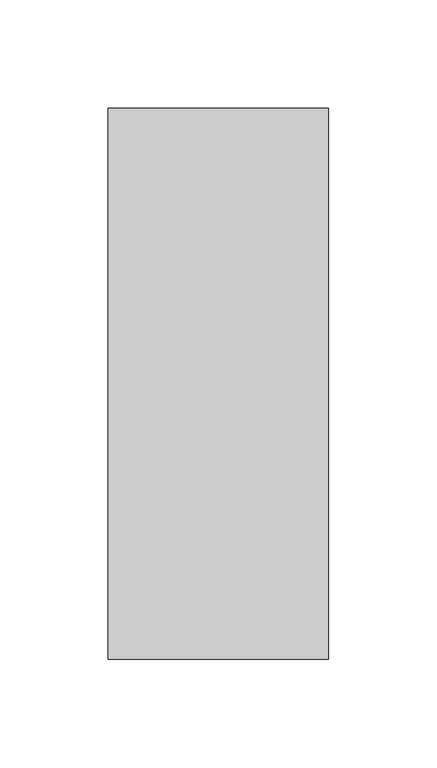
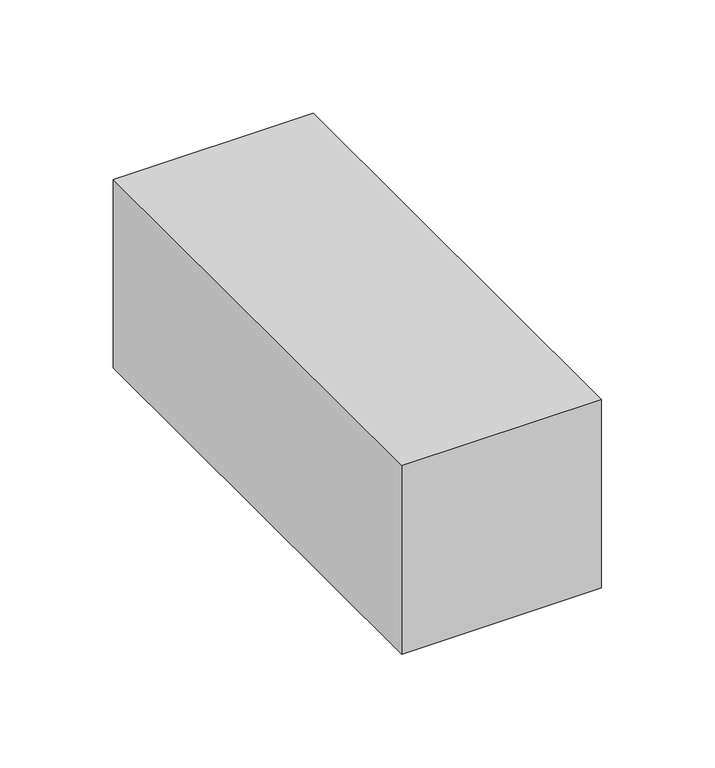
"""IFC4 building model written with IfcOpenShell, lengths in millimetres: proxy geometry, M0750 - Flowmeter, Air, Connect W50 PSI Supply : M0750 - Flowmeter, Air, Connect W50 PSI Supply."""

import ifcopenshell
import ifcopenshell.guid

model = None  # the IFC model being written
_history = None  # IfcOwnerHistory: only IFC2X3 demands one
_inside = {}  # id of a spatial element -> (the spatial element, [elements in it])
_under = {}  # id of a project, library or spatial element -> (it, [spatial elements below it])
_declared = {}  # id of a project -> (the project, [libraries it declares])
_typed = {}  # id of a type object -> (the type object, [elements of that type])
_made_of = {}  # id of a material, layer set ... -> (it, [elements and type objects made of it])


def new_model(schema):
    """Start an empty IFC model of exactly this schema.

    Asked for "IFC4X3", IfcOpenShell would pick the latest addendum, in which some entities
    have other attributes; the version numbers below select the first issue.
    IFC2X3 requires an IfcOwnerHistory on every rooted entity: one is made here for all.
    """
    global model, _history
    if schema == "IFC4X3":
        model = ifcopenshell.file(schema_version=(4, 3, 0, 0))
    else:
        model = ifcopenshell.file(schema=schema)
    _inside.clear()
    _under.clear()
    _declared.clear()
    _typed.clear()
    _made_of.clear()
    _history = None
    if model.schema == "IFC2X3":
        org = make("IfcOrganization", Name="unknown")
        user = make(
            "IfcPersonAndOrganization",
            ThePerson=make("IfcPerson", FamilyName="unknown"),
            TheOrganization=org,
        )
        app = make(
            "IfcApplication",
            ApplicationDeveloper=org,
            Version="unknown",
            ApplicationFullName="unknown",
            ApplicationIdentifier="unknown",
        )
        _history = make(
            "IfcOwnerHistory",
            OwningUser=user,
            OwningApplication=app,
            ChangeAction="ADDED",
            CreationDate=0,
        )
    return model


def make(cls, **values):
    """One entity of the class cls with the attributes given. An attribute that is None is left unset."""
    return model.create_entity(
        cls, **{name: value for name, value in values.items() if value is not None}
    )


def rooted(cls, **values):
    """An entity with a GlobalId (a new one), such as an element, a storey or a relation."""
    return make(cls, GlobalId=ifcopenshell.guid.new(), OwnerHistory=_history, **values)


def si_unit(unit_type, name, prefix=None):
    """IfcSIUnit, for example si_unit("LENGTHUNIT", "METRE", prefix="MILLI")."""
    return make("IfcSIUnit", UnitType=unit_type, Prefix=prefix, Name=name)


def assignment(units):
    """IfcUnitAssignment: the units of a project."""
    return None if units is None else make("IfcUnitAssignment", Units=units)


def point(xyz):
    """IfcCartesianPoint."""
    return None if xyz is None else make("IfcCartesianPoint", Coordinates=xyz)


def direction(xyz):
    """IfcDirection."""
    return None if xyz is None else make("IfcDirection", DirectionRatios=xyz)


def frame(location, z_axis=None, x_axis=None):
    """IfcAxis2Placement3D, a coordinate frame: its origin and axes. An axis left out is left unset."""
    return make(
        "IfcAxis2Placement3D",
        Location=point(location),
        Axis=direction(z_axis),
        RefDirection=direction(x_axis),
    )


def frame_2d(location, x_axis=None):
    """IfcAxis2Placement2D, a coordinate frame in the plane: its origin and x axis."""
    return make(
        "IfcAxis2Placement2D", Location=point(location), RefDirection=direction(x_axis)
    )


def origin():
    """The frame at (0, 0, 0) with its axes left unset."""
    return frame((0.0, 0.0, 0.0))


def origin_with_axes():
    """The frame at (0, 0, 0) with the z axis (0, 0, 1) and the x axis (1, 0, 0) written out."""
    return frame((0.0, 0.0, 0.0), z_axis=(0.0, 0.0, 1.0), x_axis=(1.0, 0.0, 0.0))


def place(relative_to, where):
    """IfcLocalPlacement: puts the frame where relative to a parent placement (None: the world)."""
    return make(
        "IfcLocalPlacement", PlacementRelTo=relative_to, RelativePlacement=where
    )


def context(
    kind, dimensions, precision=None, world=None, true_north=None, identifier=None
):
    """IfcGeometricRepresentationContext, for example the 3D "Model" context."""
    return make(
        "IfcGeometricRepresentationContext",
        ContextIdentifier=identifier,
        ContextType=kind,
        CoordinateSpaceDimension=dimensions,
        Precision=precision,
        WorldCoordinateSystem=world,
        TrueNorth=true_north,
    )


def project(units=None, contexts=None):
    """IfcProject with its units and contexts."""
    return rooted(
        "IfcProject",
        Name="project",
        RepresentationContexts=contexts,
        UnitsInContext=assignment(units),
    )


def spatial(cls, under=None, at=None, **own):
    """A site, building, storey or space (cls), placed at a placement, below another one or the project."""
    s = rooted(cls, ObjectPlacement=at, **own)
    if under is not None:
        _under.setdefault(under.id(), (under, []))[1].append(s)
    return s


def polyline(points):
    """IfcPolyline through the points."""
    return make("IfcPolyline", Points=[point(p) for p in points])


def circle_curve(where, radius):
    """IfcCircle in the frame where."""
    return make("IfcCircle", Position=where, Radius=radius)


def trimmed(basis, trim1, trim2, sense, master):
    """IfcTrimmedCurve: the piece of a basis curve between two trims."""
    return make(
        "IfcTrimmedCurve",
        BasisCurve=basis,
        Trim1=trim1,
        Trim2=trim2,
        SenseAgreement=sense,
        MasterRepresentation=master,
    )


def segment(curve, same_sense, transition):
    """IfcCompositeCurveSegment."""
    return make(
        "IfcCompositeCurveSegment",
        Transition=transition,
        SameSense=same_sense,
        ParentCurve=curve,
    )


def composite_curve(segments, self_intersect=None):
    """IfcCompositeCurve: segments joined end to end."""
    return make("IfcCompositeCurve", Segments=segments, SelfIntersect=self_intersect)


def outline(outer, holes=None, kind="AREA"):
    """IfcArbitraryClosedProfileDef: a profile drawn as a closed curve; with holes, ...WithVoids."""
    if holes is None:
        return make("IfcArbitraryClosedProfileDef", ProfileType=kind, OuterCurve=outer)
    return make(
        "IfcArbitraryProfileDefWithVoids",
        ProfileType=kind,
        OuterCurve=outer,
        InnerCurves=holes,
    )


def extrude(swept, where, along, depth):
    """IfcExtrudedAreaSolid: the profile swept, set in the frame where, extruded along a direction by depth."""
    return make(
        "IfcExtrudedAreaSolid",
        SweptArea=swept,
        Position=where,
        ExtrudedDirection=direction(along),
        Depth=depth,
    )


def shape(context_of_items, identifier, shape_type, items):
    """IfcShapeRepresentation: the items that make up one representation, for example the "Body"."""
    return make(
        "IfcShapeRepresentation",
        ContextOfItems=context_of_items,
        RepresentationIdentifier=identifier,
        RepresentationType=shape_type,
        Items=items,
    )


def source(mapping_origin, context_of_items, identifier, shape_type, items):
    """IfcRepresentationMap: a shape defined once, which mapped items show again and again."""
    return make(
        "IfcRepresentationMap",
        MappingOrigin=mapping_origin,
        MappedRepresentation=shape(context_of_items, identifier, shape_type, items),
    )


def transform(
    local_origin,
    x_axis=None,
    y_axis=None,
    z_axis=None,
    scale=None,
    scale2=None,
    scale3=None,
    uniform=True,
):
    """IfcCartesianTransformationOperator3D, or its non-uniform kind. x_axis, y_axis, z_axis: its Axis1, 2, 3."""
    if uniform:
        return make(
            "IfcCartesianTransformationOperator3D",
            Axis1=direction(x_axis),
            Axis2=direction(y_axis),
            LocalOrigin=point(local_origin),
            Scale=scale,
            Axis3=direction(z_axis),
        )
    return make(
        "IfcCartesianTransformationOperator3DnonUniform",
        Axis1=direction(x_axis),
        Axis2=direction(y_axis),
        LocalOrigin=point(local_origin),
        Scale=scale,
        Axis3=direction(z_axis),
        Scale2=scale2,
        Scale3=scale3,
    )


def mapped(mapping_source, mapping_target):
    """IfcMappedItem: shows the shape of a source again, moved by a transform."""
    return make(
        "IfcMappedItem", MappingSource=mapping_source, MappingTarget=mapping_target
    )


def made_of(thing, what):
    """Note that an element or type object is made of a material, layer set ...; save() writes the relation."""
    if what is not None:
        _made_of.setdefault(what.id(), (what, []))[1].append(thing)
    return thing


def element(
    cls,
    number,
    at=None,
    inside=None,
    cuts=None,
    type_object=None,
    material=None,
    context=None,
    identifier="Body",
    shape_type=None,
    held_by="IfcProductDefinitionShape",
    body=None,
    shapes=None,
    **own,
):
    """One element of the class cls, such as IfcWall. Its Tag is "e" and its number.

    at: its placement. inside: the storey or other place that contains it. cuts: it is an
    opening in that element (IfcRelVoidsElement). A single representation is given by context,
    identifier, shape_type and body (its items); several are given by shapes. held_by: the class
    of the entity that holds the representations. save() writes the other relations.
    """
    e = rooted(cls, Tag="e%d" % number, ObjectPlacement=at, **own)
    if body is not None:
        shapes = [shape(context, identifier, shape_type, body)]
    if shapes is not None:
        e.Representation = make(held_by, Representations=shapes)
    if inside is not None:
        _inside.setdefault(inside.id(), (inside, []))[1].append(e)
    if cuts is not None:
        rooted(
            "IfcRelVoidsElement", RelatingBuildingElement=cuts, RelatedOpeningElement=e
        )
    if type_object is not None:
        _typed.setdefault(type_object.id(), (type_object, []))[1].append(e)
    return made_of(e, material)


def aggregate(whole, parts):
    """IfcRelAggregates: a whole, such as a stair, and the parts it consists of."""
    return rooted("IfcRelAggregates", RelatingObject=whole, RelatedObjects=parts)


def save(model, path):
    """Write the relations noted so far, then the file.

    IfcRelAggregates (storeys below a building ...), IfcRelContainedInSpatialStructure (elements
    in a storey), IfcRelDefinesByType, IfcRelAssociatesMaterial and IfcRelDeclares: one each for
    every whole, place, type object, material and project.
    """
    for whole, parts in _under.values():
        aggregate(whole, parts)
    for where, things in _inside.values():
        rooted(
            "IfcRelContainedInSpatialStructure",
            RelatedElements=things,
            RelatingStructure=where,
        )
    for kind, things in _typed.values():
        rooted("IfcRelDefinesByType", RelatedObjects=things, RelatingType=kind)
    for what, things in _made_of.values():
        rooted("IfcRelAssociatesMaterial", RelatedObjects=things, RelatingMaterial=what)
    for by, libraries in _declared.values():
        rooted("IfcRelDeclares", RelatingContext=by, RelatedDefinitions=libraries)
    model.write(path)


def plane_surface(at):
    """IfcPlane: the flat surface through the origin of the frame at, square to its z axis."""
    return make("IfcPlane", Position=at)


def cylinder_surface(at, radius):
    """IfcCylindricalSurface: all points at the distance radius from the z axis of the frame at."""
    return make("IfcCylindricalSurface", Position=at, Radius=radius)


def revolved_surface(curve, axis_point, axis_direction):
    """IfcSurfaceOfRevolution: the curve turned about the line through axis_point along axis_direction."""
    return make(
        "IfcSurfaceOfRevolution",
        SweptCurve=make("IfcArbitraryOpenProfileDef", ProfileType="CURVE", Curve=curve),
        AxisPosition=make("IfcAxis1Placement", Location=point(axis_point), Axis=direction(axis_direction)),
    )


def advanced_brep(points, edges, surfaces, faces):
    """IfcAdvancedBrep: a solid bounded by faces that lie on surfaces and meet in shared edges.

    An edge is (start, end): straight between two places in points (the first is 0);
    or (start, end, curve); or (start, end, curve, False) where it runs against its curve.
    A face is (place in surfaces, loops), or (place, loops, False) where it looks against
    its surface's normal. A loop lists edges by number (the first is 1), with a minus sign
    where the edge is run from its end to its start. The first loop is the outer one.
    """
    corners = [point(p) for p in points]
    vertices = [make("IfcVertexPoint", VertexGeometry=c) for c in corners]
    made = []
    for start, end, *more in edges:
        made.append(
            make(
                "IfcEdgeCurve",
                EdgeStart=vertices[start],
                EdgeEnd=vertices[end],
                EdgeGeometry=more[0] if more else make("IfcPolyline", Points=[corners[start], corners[end]]),
                SameSense=more[1] if len(more) > 1 else True,
            )
        )
    hull = []
    for where, loops, *sense in faces:
        bounds = []
        for j, loop in enumerate(loops):
            ring = [make("IfcOrientedEdge", EdgeElement=made[abs(k) - 1], Orientation=k > 0) for k in loop]
            bounds.append(
                make(
                    "IfcFaceOuterBound" if j == 0 else "IfcFaceBound",
                    Bound=make("IfcEdgeLoop", EdgeList=ring),
                    Orientation=True,
                )
            )
        hull.append(make("IfcAdvancedFace", Bounds=bounds, FaceSurface=surfaces[where], SameSense=sense[0] if sense else True))
    return make("IfcAdvancedBrep", Outer=make("IfcClosedShell", CfsFaces=hull))


def specialty_equipment_dfd23612(model_context):
    return source(origin(), model_context, "Body", "SolidModel", [
        extrude(outline(polyline([(-50.8, -254.0), (-50.8, 0.0), (50.8, 0.0), (50.8, -254.0), (-50.8, -254.0)])), origin_with_axes(), (0.0, 0.0, 1.0), 101.6),
        extrude(outline(composite_curve([segment(trimmed(circle_curve(frame_2d((0.0, -43.7511243)), 11.1125), [point((-11.1125, -43.7511243))], [point((11.1125, -43.7511243))], False, "CARTESIAN"), True, "CONTINUOUS"), segment(trimmed(circle_curve(frame_2d((0.0, -43.7511243)), 11.1125), [point((11.1125, -43.7511243))], [point((-11.1125, -43.7511243))], False, "CARTESIAN"), True, "CONTINUOUS")], self_intersect=False)), origin_with_axes(), (0.0, 0.0, 1.0), 12.1432676),
        extrude(outline(composite_curve([segment(trimmed(circle_curve(frame_2d((0.0, -43.7511243)), 6.35), [point((-6.35, -43.7511243))], [point((6.35, -43.7511243))], False, "CARTESIAN"), True, "CONTINUOUS"), segment(trimmed(circle_curve(frame_2d((0.0, -43.7511243)), 6.35), [point((6.35, -43.7511243))], [point((-6.35, -43.7511243))], False, "CARTESIAN"), True, "CONTINUOUS")], self_intersect=False)), frame((0.0, 0.0, 12.1432676), z_axis=(0.0, 0.0, 1.0), x_axis=(1.0, 0.0, 0.0)), (0.0, 0.0, 1.0), 11.6740858),
        extrude(outline(composite_curve([segment(trimmed(circle_curve(frame_2d((0.0, -43.7511243)), 11.1125), [point((-11.1125, -43.7511243))], [point((11.1125, -43.7511243))], False, "CARTESIAN"), True, "CONTINUOUS"), segment(trimmed(circle_curve(frame_2d((0.0, -43.7511243)), 11.1125), [point((11.1125, -43.7511243))], [point((-11.1125, -43.7511243))], False, "CARTESIAN"), True, "CONTINUOUS")], self_intersect=False)), frame((0.0, 0.0, 12.8429111), z_axis=(0.0, 0.0, 1.0), x_axis=(1.0, 0.0, 0.0)), (0.0, 0.0, 1.0), 3.7345018),
        advanced_brep(
        [(0.0, -195.0035492, 41.6430751), (0.0, -195.0035492, 28.9430751), (0.0, -77.2962509, 43.2305751), (0.0, -77.2962509, 27.3555751)],
        [
            (0, 1, circle_curve(frame((0.0, -195.0035492, 35.2930751), z_axis=(0.0, -1.0, 0.0), x_axis=(0.0, 0.0, -1.0)), 6.35)),
            (1, 0, circle_curve(frame((0.0, -195.0035492, 35.2930751), z_axis=(0.0, -1.0, 0.0), x_axis=(0.0, 0.0, 1.0)), 6.35)),
            (2, 3, circle_curve(frame((0.0, -77.2962509, 35.2930751), z_axis=(0.0, 1.0, 0.0), x_axis=(0.0, 0.0, 1.0)), 7.9375)),
            (3, 2, circle_curve(frame((0.0, -77.2962509, 35.2930751), z_axis=(0.0, 1.0, 0.0), x_axis=(0.0, 0.0, -1.0)), 7.9375)),
            (2, 0),
            (1, 3),
        ],
        [
            plane_surface(frame((0.0, -195.0035492, 35.2930751), z_axis=(0.0, -1.0, 0.0), x_axis=(1.0, 0.0, 0.0))),
            plane_surface(frame((0.0, -77.2962509, 35.2930751), z_axis=(0.0, 1.0, 0.0), x_axis=(1.0, 0.0, 0.0))),
            revolved_surface(polyline([(0.0, -195.0035492, 41.64307510053948), (0.0, -77.29625090000002, 43.2305751)]), (0.0, -665.8327426, 35.2930751), (0.0, 1.0, 0.0)),
            revolved_surface(polyline([(0.0, -195.0035492, 28.943075099460525), (0.0, -77.29625090000002, 27.3555751)]), (0.0, -665.8327426, 35.2930751), (0.0, 1.0, 0.0)),
        ],
        [
            (0, [[1, 2]]),
            (1, [[3, 4]]),
            (2, [[5, -2, 6, -3]]),
            (3, [[-6, -1, -5, -4]]),
        ],
    ),
        extrude(outline(composite_curve([segment(trimmed(circle_curve(frame_2d((0.0, -56.2938544)), 15.875), [point((-15.875, -56.2938544))], [point((15.875, -56.2938544))], False, "CARTESIAN"), True, "CONTINUOUS"), segment(trimmed(circle_curve(frame_2d((0.0, -56.2938544)), 15.875), [point((15.875, -56.2938544))], [point((-15.875, -56.2938544))], False, "CARTESIAN"), True, "CONTINUOUS")], self_intersect=False)), frame((0.0, 0.0, 73.7139717), z_axis=(0.0, 0.0, 1.0), x_axis=(1.0, 0.0, 0.0)), (0.0, 0.0, 1.0), 9.1021363),
        advanced_brep(
        [(0.0, -197.9462509, 44.8180751), (0.0, -197.9462509, 25.7680751), (0.0, -77.2962509, 46.4055751), (0.0, -77.2962509, 24.1805751)],
        [
            (0, 1, circle_curve(frame((0.0, -197.9462509, 35.2930751), z_axis=(0.0, -1.0, 0.0), x_axis=(0.0, 0.0, -1.0)), 9.525)),
            (1, 0, circle_curve(frame((0.0, -197.9462509, 35.2930751), z_axis=(0.0, -1.0, 0.0), x_axis=(0.0, 0.0, 1.0)), 9.525)),
            (2, 3, circle_curve(frame((0.0, -77.2962509, 35.2930751), z_axis=(0.0, 1.0, 0.0), x_axis=(0.0, 0.0, 1.0)), 11.1125)),
            (3, 2, circle_curve(frame((0.0, -77.2962509, 35.2930751), z_axis=(0.0, 1.0, 0.0), x_axis=(0.0, 0.0, -1.0)), 11.1125)),
            (2, 0),
            (1, 3),
        ],
        [
            plane_surface(frame((0.0, -197.9462509, 35.2930751), z_axis=(0.0, -1.0, 0.0), x_axis=(1.0, 0.0, 0.0))),
            plane_surface(frame((0.0, -77.2962509, 35.2930751), z_axis=(0.0, 1.0, 0.0), x_axis=(1.0, 0.0, 0.0))),
            revolved_surface(polyline([(0.0, -197.9462509, 44.8180751), (0.0, -77.29625090000002, 46.4055751)]), (0.0, -921.8462509, 35.2930751), (0.0, 1.0, 0.0)),
            revolved_surface(polyline([(0.0, -197.9462509, 25.768075099999997), (0.0, -77.29625090000002, 24.1805751)]), (0.0, -921.8462509, 35.2930751), (0.0, 1.0, 0.0)),
        ],
        [
            (0, [[1, 2]]),
            (1, [[3, 4]]),
            (2, [[5, -2, 6, -3]]),
            (3, [[-6, -1, -5, -4]]),
        ],
    ),
        advanced_brep(
        [(16.4405012, -77.2962509, 35.2930751), (0.0, -77.2962509, 35.2930751), (-16.4405012, -77.2962509, 35.2930751), (17.4336479, -76.3031042, 35.2930751), (-17.4336479, -76.3031042, 35.2930751), (17.4336479, -64.5962509, 35.2930751), (-17.4336479, -64.5962509, 35.2930751), (14.6960919, -64.5962509, 35.2930751), (-14.6960919, -64.5962509, 35.2930751), (14.6960919, -63.5321613, 35.2930751), (-14.6960919, -63.5321613, 35.2930751), (15.9348033, -63.5321613, 35.2930751), (-15.9348033, -63.5321613, 35.2930751), (15.9348033, -33.3696613, 35.2930751), (-15.9348033, -33.3696613, 35.2930751), (8.893951, -30.7772209, 35.2930751), (-8.893951, -30.7772209, 35.2930751), (4.4469755, -30.7772209, 35.2930751), (-4.4469755, -30.7772209, 35.2930751), (4.4469755, -25.4, 35.2930751), (-4.4469755, -25.4, 35.2930751), (0.0, -25.4, 35.2930751)],
        [
            (0, 1),
            (1, 2),
            (2, 0, circle_curve(frame((0.0, -77.2962509, 35.2930751), z_axis=(0.0, -1.0, 0.0), x_axis=(-1.0, 0.0, 0.0)), 16.4405012)),
            (0, 2, circle_curve(frame((0.0, -77.2962509, 35.2930751), z_axis=(0.0, -1.0, 0.0), x_axis=(-1.0, 0.0, 0.0)), 16.4405012)),
            (3, 0),
            (2, 4),
            (4, 3, circle_curve(frame((0.0, -76.3031042, 35.2930751), z_axis=(0.0, -1.0, 0.0), x_axis=(-1.0, 0.0, 0.0)), 17.4336479)),
            (3, 4, circle_curve(frame((0.0, -76.3031042, 35.2930751), z_axis=(0.0, -1.0, 0.0), x_axis=(-1.0, 0.0, 0.0)), 17.4336479)),
            (5, 3),
            (4, 6),
            (6, 5, circle_curve(frame((0.0, -64.5962509, 35.2930751), z_axis=(0.0, -1.0, 0.0), x_axis=(-1.0, 0.0, 0.0)), 17.4336479)),
            (5, 6, circle_curve(frame((0.0, -64.5962509, 35.2930751), z_axis=(0.0, -1.0, 0.0), x_axis=(-1.0, 0.0, 0.0)), 17.4336479)),
            (7, 5),
            (6, 8),
            (8, 7, circle_curve(frame((0.0, -64.5962509, 35.2930751), z_axis=(0.0, -1.0, 0.0), x_axis=(-1.0, 0.0, 0.0)), 14.6960919)),
            (7, 8, circle_curve(frame((0.0, -64.5962509, 35.2930751), z_axis=(0.0, -1.0, 0.0), x_axis=(-1.0, 0.0, 0.0)), 14.6960919)),
            (9, 7),
            (8, 10),
            (10, 9, circle_curve(frame((0.0, -63.5321613, 35.2930751), z_axis=(0.0, -1.0, 0.0), x_axis=(-1.0, 0.0, 0.0)), 14.6960919)),
            (9, 10, circle_curve(frame((0.0, -63.5321613, 35.2930751), z_axis=(0.0, -1.0, 0.0), x_axis=(-1.0, 0.0, 0.0)), 14.6960919)),
            (11, 9),
            (10, 12),
            (12, 11, circle_curve(frame((0.0, -63.5321613, 35.2930751), z_axis=(0.0, -1.0, 0.0), x_axis=(-1.0, 0.0, 0.0)), 15.9348033)),
            (11, 12, circle_curve(frame((0.0, -63.5321613, 35.2930751), z_axis=(0.0, -1.0, 0.0), x_axis=(-1.0, 0.0, 0.0)), 15.9348033)),
            (13, 11),
            (12, 14),
            (14, 13, circle_curve(frame((0.0, -33.3696613, 35.2930751), z_axis=(0.0, -1.0, 0.0), x_axis=(-1.0, 0.0, 0.0)), 15.9348033)),
            (13, 14, circle_curve(frame((0.0, -33.3696613, 35.2930751), z_axis=(0.0, -1.0, 0.0), x_axis=(-1.0, 0.0, 0.0)), 15.9348033)),
            (15, 13),
            (14, 16),
            (16, 15, circle_curve(frame((0.0, -30.7772209, 35.2930751), z_axis=(0.0, -1.0, 0.0), x_axis=(-1.0, 0.0, 0.0)), 8.893951)),
            (15, 16, circle_curve(frame((0.0, -30.7772209, 35.2930751), z_axis=(0.0, -1.0, 0.0), x_axis=(-1.0, 0.0, 0.0)), 8.893951)),
            (17, 15),
            (16, 18),
            (18, 17, circle_curve(frame((0.0, -30.7772209, 35.2930751), z_axis=(0.0, -1.0, 0.0), x_axis=(-1.0, 0.0, 0.0)), 4.4469755)),
            (17, 18, circle_curve(frame((0.0, -30.7772209, 35.2930751), z_axis=(0.0, -1.0, 0.0), x_axis=(-1.0, 0.0, 0.0)), 4.4469755)),
            (19, 17),
            (18, 20),
            (20, 19, circle_curve(frame((0.0, -25.4, 35.2930751), z_axis=(0.0, -1.0, 0.0), x_axis=(-1.0, 0.0, 0.0)), 4.4469755)),
            (19, 20, circle_curve(frame((0.0, -25.4, 35.2930751), z_axis=(0.0, -1.0, 0.0), x_axis=(-1.0, 0.0, 0.0)), 4.4469755)),
            (21, 19),
            (20, 21),
        ],
        [
            plane_surface(frame((0.0, -77.2962509, 35.2930751), z_axis=(0.0, -1.0, 0.0), x_axis=(-1.0, 0.0, 0.0))),
            revolved_surface(polyline([(-16.4405012, -77.2962509, 35.2930751), (-17.4336479, -76.3031042, 35.2930751)]), (0.0, -77.2962509, 35.2930751), (0.0, 1.0, 0.0)),
            cylinder_surface(frame((0.0, -77.2962509, 35.2930751), z_axis=(0.0, 1.0, 0.0), x_axis=(-1.0, 0.0, 0.0)), 17.4336479),
            plane_surface(frame((0.0, -64.5962509, 35.2930751), z_axis=(0.0, 1.0, 0.0), x_axis=(-1.0, 0.0, 0.0))),
            cylinder_surface(frame((0.0, -77.2962509, 35.2930751), z_axis=(0.0, 1.0, 0.0), x_axis=(-1.0, 0.0, 0.0)), 14.6960919),
            plane_surface(frame((0.0, -63.5321613, 35.2930751), z_axis=(0.0, -1.0, 0.0), x_axis=(-1.0, 0.0, 0.0))),
            cylinder_surface(frame((0.0, -77.2962509, 35.2930751), z_axis=(0.0, 1.0, 0.0), x_axis=(-1.0, 0.0, 0.0)), 15.9348033),
            revolved_surface(polyline([(-15.9348033, -33.3696613, 35.2930751), (-8.893951, -30.7772209, 35.2930751)]), (0.0, -77.2962509, 35.2930751), (0.0, 1.0, 0.0)),
            plane_surface(frame((0.0, -30.7772209, 35.2930751), z_axis=(0.0, 1.0, 0.0), x_axis=(-1.0, 0.0, 0.0))),
            cylinder_surface(frame((0.0, -77.2962509, 35.2930751), z_axis=(0.0, 1.0, 0.0), x_axis=(-1.0, 0.0, 0.0)), 4.4469755),
            plane_surface(frame((0.0, -25.4, 35.2930751), z_axis=(0.0, 1.0, 0.0), x_axis=(-1.0, 0.0, 0.0))),
        ],
        [
            (0, [[1, 2, 3]]),
            (0, [[-2, -1, 4]]),
            (1, [[5, -3, 6, 7]]),
            (1, [[-6, -4, -5, 8]]),
            (2, [[9, -7, 10, 11]]),
            (2, [[-10, -8, -9, 12]]),
            (3, [[13, -11, 14, 15]]),
            (3, [[-14, -12, -13, 16]]),
            (4, [[17, -15, 18, 19]]),
            (4, [[-18, -16, -17, 20]]),
            (5, [[21, -19, 22, 23]]),
            (5, [[-22, -20, -21, 24]]),
            (6, [[25, -23, 26, 27]]),
            (6, [[-26, -24, -25, 28]]),
            (7, [[29, -27, 30, 31]]),
            (7, [[-30, -28, -29, 32]]),
            (8, [[33, -31, 34, 35]]),
            (8, [[-34, -32, -33, 36]]),
            (9, [[37, -35, 38, 39]]),
            (9, [[-38, -36, -37, 40]]),
            (10, [[41, -39, 42]]),
            (10, [[-42, -40, -41]]),
        ],
    ),
        extrude(outline(composite_curve([segment(trimmed(circle_curve(frame_2d((0.0, -56.2938544)), 4.7625), [point((-4.7625, -56.2938544))], [point((4.7625, -56.2938544))], False, "CARTESIAN"), True, "CONTINUOUS"), segment(trimmed(circle_curve(frame_2d((0.0, -56.2938544)), 4.7625), [point((4.7625, -56.2938544))], [point((-4.7625, -56.2938544))], False, "CARTESIAN"), True, "CONTINUOUS")], self_intersect=False)), frame((0.0, 0.0, 50.024421), z_axis=(0.0, 0.0, 1.0), x_axis=(1.0, 0.0, 0.0)), (0.0, 0.0, 1.0), 33.6662415),
        extrude(outline(polyline([(-4.0213654, -63.2590636), (-8.0427308, -56.2938544), (-4.0213654, -49.3286452), (4.0213654, -49.3286452), (8.0427308, -56.2938544), (4.0213654, -63.2590636), (-4.0213654, -63.2590636)])), frame((0.0, 0.0, 54.0167391), z_axis=(0.0, 0.0, 1.0), x_axis=(1.0, 0.0, 0.0)), (0.0, 0.0, 1.0), 12.0291395),
        advanced_brep(
        [(5.8611698, -21.8455296, 35.2930751), (5.8611698, -25.4, 35.2930751), (-5.8611698, -25.4, 35.2930751), (-5.8611698, -21.8455296, 35.2930751), (2.0092135, 0.0, 35.2930751), (-2.0092135, 0.0, 35.2930751), (0.0, 0.0, 35.2930751), (0.0, -25.4, 35.2930751)],
        [
            (0, 1),
            (1, 2, circle_curve(frame((0.0, -25.4, 35.2930751), z_axis=(0.0, 1.0, 0.0), x_axis=(-1.0, 0.0, 0.0)), 5.8611698)),
            (2, 3),
            (3, 0, circle_curve(frame((0.0, -21.8455296, 35.2930751), z_axis=(0.0, -1.0, 0.0), x_axis=(-1.0, 0.0, 0.0)), 5.8611698)),
            (2, 1, circle_curve(frame((0.0, -25.4, 35.2930751), z_axis=(0.0, 1.0, 0.0), x_axis=(-1.0, 0.0, 0.0)), 5.8611698)),
            (0, 3, circle_curve(frame((0.0, -21.8455296, 35.2930751), z_axis=(0.0, -1.0, 0.0), x_axis=(-1.0, 0.0, 0.0)), 5.8611698)),
            (4, 0),
            (3, 5),
            (5, 4, circle_curve(frame((0.0, 0.0, 35.2930751), z_axis=(0.0, -1.0, 0.0), x_axis=(-1.0, 0.0, 0.0)), 2.0092135)),
            (4, 5, circle_curve(frame((0.0, 0.0, 35.2930751), z_axis=(0.0, -1.0, 0.0), x_axis=(-1.0, 0.0, 0.0)), 2.0092135)),
            (6, 4),
            (5, 6),
            (1, 7),
            (7, 2),
        ],
        [
            cylinder_surface(frame((0.0, -23.4018459, 35.2930751), z_axis=(0.0, 1.0, 0.0), x_axis=(-1.0, 0.0, 0.0)), 5.8611698),
            revolved_surface(polyline([(-5.8611698, -21.8455296, 35.2930751), (-2.0092135, 0.0, 35.2930751)]), (0.0, -23.4018459, 35.2930751), (0.0, 1.0, 0.0)),
            plane_surface(frame((0.0, 0.0, 35.2930751), z_axis=(0.0, 1.0, 0.0), x_axis=(-1.0, 0.0, 0.0))),
            plane_surface(frame((0.0, -25.4, 35.2930751), z_axis=(0.0, -1.0, 0.0), x_axis=(-1.0, 0.0, 0.0))),
        ],
        [
            (0, [[1, 2, 3, 4]]),
            (0, [[-3, 5, -1, 6]]),
            (1, [[7, -4, 8, 9]]),
            (1, [[-8, -6, -7, 10]]),
            (2, [[11, -9, 12]]),
            (2, [[-12, -10, -11]]),
            (3, [[13, 14, -2]]),
            (3, [[-14, -13, -5]]),
        ],
    ),
    ])


if __name__ == "__main__":
    model = new_model("IFC4")
    model_context = context("Model", 3, world=origin())
    ifc_project = project(units=[si_unit("LENGTHUNIT", "METRE", prefix="MILLI")], contexts=[model_context])
    site = spatial("IfcSite", under=ifc_project)
    building = spatial("IfcBuilding", under=site)
    placement = place(None, origin())
    specialty_equipment_shape = specialty_equipment_dfd23612(model_context)
    element("IfcBuildingElementProxy", 1, Name="M0750 - Flowmeter, Air, Connect W50 PSI Supply : M0750 - Flowmeter, Air, Connect W50 PSI Supply", ObjectType="M0750 - Flowmeter, Air, Connect W50 PSI Supply : M0750 - Flowmeter, Air, Connect W50 PSI Supply", at=placement, inside=building, context=model_context, shape_type="MappedRepresentation", body=[
        mapped(specialty_equipment_shape, transform((0.0, 0.0, 0.0), x_axis=(1.0, 0.0, 0.0), y_axis=(0.0, 1.0, 0.0), z_axis=(0.0, 0.0, 1.0))),
    ])
    save(model, "model.ifc")

# Revit data of these elements
# Type "M0750 - Flowmeter, Air, Connect W50 PSI Supply : M0750 - Flowmeter, Air, Connect W50 PSI Supply"
#   Watts2 = "0"
#   Watts1 = "0"
#   Unit_Issue = "EA"
#   UTIL_6_Misc = "-"
#   UTIL_5_NonMedGas = "-"
#   UTIL_4_MiscGas = "-"
#   UTIL_3_MedGas = "K"
#   UTIL_2_Elec = "-"
#   UTIL_1_WaterDrain = "-"
#   Nomenclature = "Flowmeter, Air, Connect w/50 PSI Supply"
#   NSN = "6530"
#   Location [instance default] = ""
#   JSN = "M0750"
#   Fund_Source_VA = "-"
#   Fund_Source_Navy = "-"
#   Fund_Source_Army = "-"
#   Fund_Source_AF = "-"
#   ELEC_Volts2 = "0"
#   ELEC_Volts1 = "0"
#   ELEC_Phase2 = "0"
#   ELEC_Phase1 = "0"
#   ELEC_HertzSwitch = "0"
#   ELEC_HertzDependent = "0"
#   ELEC_Hertz = "0"
#   ELEC_Amps2 = "0"
#   ELEC_Amps1 = "0"
#   DetailDescription = "Air flowmeter. Unit has a stainless steel needle valve with clear flowtube for connection to 50 PSI air outlet from central pipeline system. Requires the appropriate adapter for connection to the wall outlet and fitting to connect to tubing. Database prices reflect fittings with an attached DISS power outlet. Other outlet and adapter configurations are available."
#   CAT_VA = "C"
#   CAT_Navy = "C"
#   CAT_IHS = "-"
#   CAT_Army = "C"
#   CAT_AF = "C"
#   BTUperhour = "0"
#   Weight_IP = 3
#   Default Elevation = 4' - 0"
#   DIM_Width_IP = 0' - 4"
#   DIM_Height_IP = 0' - 10"
#   DIM_Depth_IP = 0' - 4"
#   finish [instance default] = none
# Element 1 (IfcBuildingElementProxy, "M0750 - Flowmeter, Air, Connect W50 PSI Supply : M0750 - Flowmeter, Air, Connect W50 PSI Supply")
#   Materials on its faces: "Glass", "EquipSpace"
# Materials
#   "Glass": class "Glass", colour RGB 0 128 192, transparency 0.75
#   "EquipSpace": class "Unassigned", colour RGB 221 217 195, transparency 0.5
